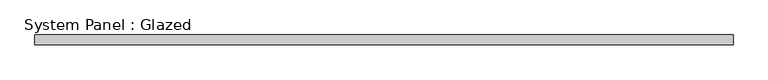
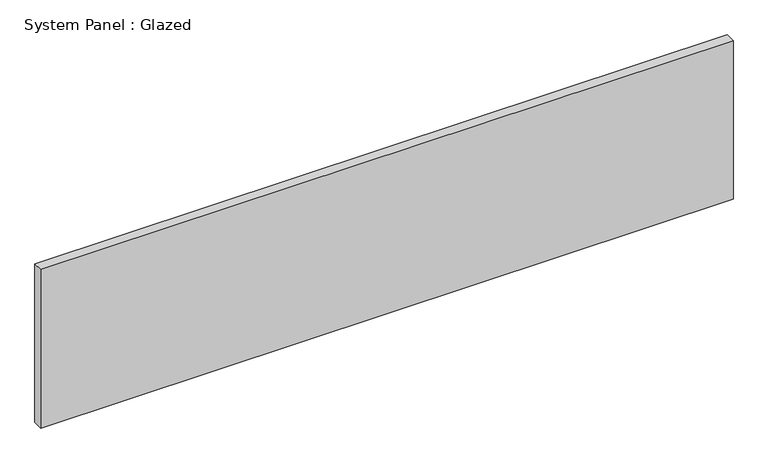
"""IFC4 building model written with IfcOpenShell, lengths in millimetres: plate geometry, System Panel : Glazed."""

from ifc_helpers import new_model, si_unit, origin, origin_with_axes, place, context, project, spatial, polyline, outline, extrude, source, transform, mapped, element, save


def system_panel_glazed_66e2820e(model_context):
    return source(origin(), model_context, "Body", "SweptSolid", [
        extrude(outline(polyline([(877.5, -49.5), (-877.5, -49.5), (-877.5, -24.5), (877.5, -24.5), (877.5, -49.5)])), origin_with_axes(), (0.0, 0.0, 1.0), 425.0),
    ])


if __name__ == "__main__":
    model = new_model("IFC4")
    model_context = context("Model", 3, world=origin())
    ifc_project = project(units=[si_unit("LENGTHUNIT", "METRE", prefix="MILLI")], contexts=[model_context])
    site = spatial("IfcSite", under=ifc_project)
    building = spatial("IfcBuilding", under=site)
    placement = place(None, origin())
    system_panel_glazed_shape = system_panel_glazed_66e2820e(model_context)
    element("IfcPlate", 1, ObjectType="System Panel : Glazed", at=placement, inside=building, context=model_context, shape_type="MappedRepresentation", body=[
        mapped(system_panel_glazed_shape, transform((0.0, 0.0, 0.0), x_axis=(1.0, 0.0, 0.0), y_axis=(0.0, 1.0, 0.0), z_axis=(0.0, 0.0, 1.0))),
    ])
    save(model, "model.ifc")

# Revit data of these elements
# Type "System Panel : Glazed"
#   Keynote = "H11"
#   Construction Type Id = "GSP4R"
#   Analytic Construction = "1/8 in Pilkington single glazing"
#   Visual Light Transmittance = 0.9
#   Solar Heat Gain Coefficient = 0.86
#   Heat Transfer Coefficient (U) = 6.7069 W/(m²·K)
# Element 1 (IfcPlate, "System Panel : Glazed")
#   Materials on its faces: "Glass"
# Materials
#   "Glass": class "Glass", colour RGB 0 128 192, transparency 0.9, Description = "Soda Lime Glass", Cost = 0
